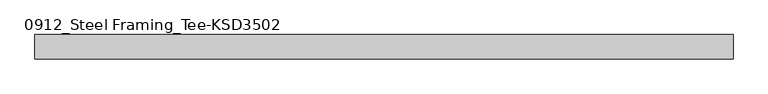
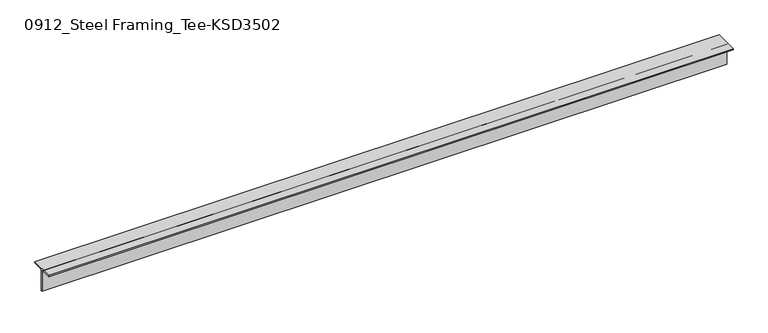
"""IFC4 building model written with IfcOpenShell, lengths in millimetres: member geometry, 0912_Steel Framing_Tee-KSD3502 : H_SB_ASB_CT-150x150x6.5x9."""

from ifc_helpers import new_model, si_unit, point, frame, frame_2d, origin, place, context, project, spatial, polyline, circle_curve, trimmed, segment, composite_curve, outline, extrude, source, transform, mapped, element, save


def member_0912_steel_framing_tee_ksd3502_d47455c7(model_context):
    return source(origin(), model_context, "Body", "SweptSolid", [
        extrude(outline(composite_curve([segment(polyline([(-75.0, 75.0), (75.0, 75.0), (75.0, 66.0), (16.25, 66.0)]), True, "CONTINUOUS"), segment(trimmed(circle_curve(frame_2d((16.25, 53.0)), 13.0), [point((16.25, 66.0))], [point((3.25, 53.0))], True, "CARTESIAN"), True, "CONTINUOUS"), segment(polyline([(3.25, 53.0), (3.25, -75.0), (-3.25, -75.0), (-3.25, 53.0)]), True, "CONTINUOUS"), segment(trimmed(circle_curve(frame_2d((-16.25, 53.0)), 13.0), [point((-3.25, 53.0))], [point((-16.25, 66.0))], True, "CARTESIAN"), True, "CONTINUOUS"), segment(polyline([(-16.25, 66.0), (-75.0, 66.0), (-75.0, 75.0)]), True, "CONTINUOUS")], self_intersect=False)), frame((-2227.6, 0.0, 0.0), z_axis=(1.0, 0.0, 0.0), x_axis=(0.0, 1.0, 0.0)), (0.0, 0.0, 1.0), 4330.1),
    ])


if __name__ == "__main__":
    model = new_model("IFC4")
    model_context = context("Model", 3, world=origin())
    ifc_project = project(units=[si_unit("LENGTHUNIT", "METRE", prefix="MILLI")], contexts=[model_context])
    site = spatial("IfcSite", under=ifc_project)
    building = spatial("IfcBuilding", under=site)
    placement = place(None, origin())
    member_0912_steel_framing_tee_ksd3502_shape = member_0912_steel_framing_tee_ksd3502_d47455c7(model_context)
    element("IfcMember", 1, ObjectType="0912_Steel Framing_Tee-KSD3502 : H_SB_ASB_CT-150x150x6.5x9", at=placement, inside=building, context=model_context, shape_type="MappedRepresentation", body=[
        mapped(member_0912_steel_framing_tee_ksd3502_shape, transform((0.0, 0.0, 0.0), x_axis=(1.0, 0.0, 0.0), y_axis=(0.0, 1.0, 0.0), z_axis=(0.0, 0.0, 1.0))),
    ])
    save(model, "model.ifc")

# Revit data of these elements
# Type "0912_Steel Framing_Tee-KSD3502 : H_SB_ASB_CT-150x150x6.5x9"
#   H_WM Code_1 = "S01AA003-00001 | Main Steel Structure Fabrication Work | Shelter/Building | Light Steel - Standard (30KG/M>Weight) | Material: (   )"
#   H_WM Code_2 = "S03AA029-00001 | Main Steel Structure Erection Work | Shelter/Building | Light Steel (30KG/M>Weight) | Material: (   )"
#   H_WM Code_3 = "S01AA010-00001 | Main Steel Structure Fabrication Work | Shelter/Building | Steel Painting/Coating | for Non-Fireproofed Steel Surface, Surface Preparation, Primer, Second & Final Coat | Material: (   )"
#   H_Q'ty Cal Type Tag = "SB-Q2"
#   Width = 15.0 cm
#   Web Thickness = 0.65 cm
#   Web Fillet = 1.3 cm
#   Section Area = 23.39 cm²
#   Perimeter = 0.60 m²/m
#   Nominal Weight = 18.40 kgf/m
#   Height = 15.0 cm
#   Flange Thickness = 0.9 cm
#   Centroid Vertical = 7.5 cm
#   Centroid Horizontal = 7.5 cm
#   Length [instance default] = 1.5000 m
#   Structural Material [instance default] = Steel, 45-345
#   Warping Constant = (empty or 0)
#   Torsional Moment of Inertia = 0
#   Section Name Key = ""
#   Plastic Modulus weak axis = 0
#   Plastic Modulus strong axis = 0
#   Moment of Inertia weak axis = 0
#   Moment of Inertia strong axis = 0
#   Elastic Modulus weak axis = 0
#   Elastic Modulus strong axis = 0
#   Bolt Spacing = 0
#   Assembly Code = ""
# Element 1 (IfcMember, "0912_Steel Framing_Tee-KSD3502 : H_SB_ASB_CT-150x150x6.5x9")
#   Structural Material = none
# Materials
#   "Steel, 45-345": class "Metal", colour RGB 189 187 185, transparency 0, Description = "Steel 345 MPa", Cost = 0
